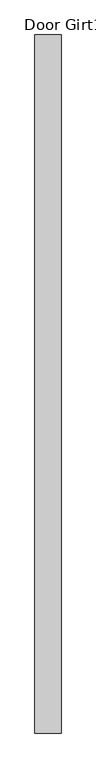
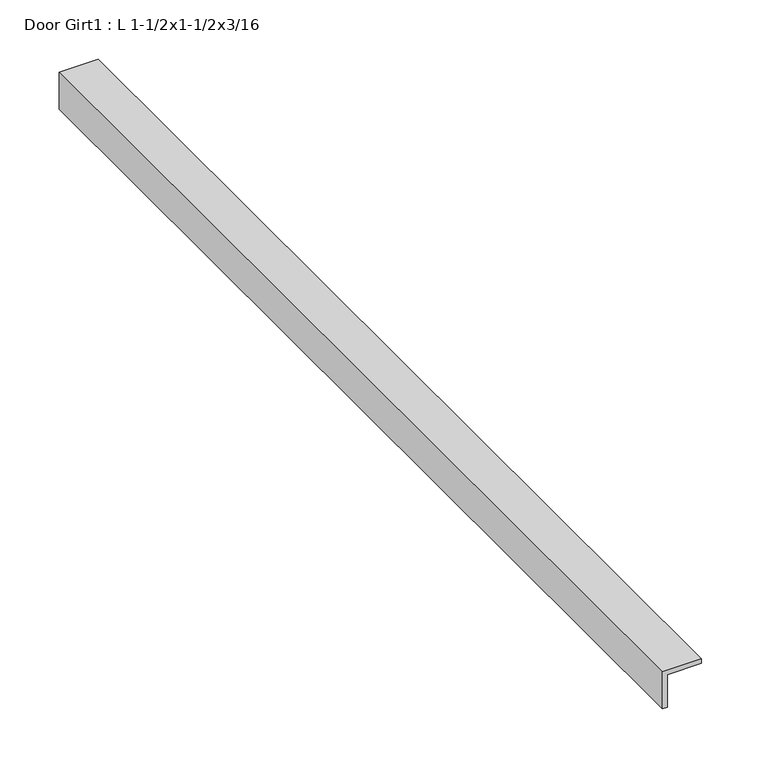
"""IFC4 building model written with IfcOpenShell, lengths in millimetres: proxy geometry, Door Girt1 : L 1-1/2x1-1/2x3/16."""

import ifcopenshell
import ifcopenshell.guid

model = None  # the IFC model being written
_history = None  # IfcOwnerHistory: only IFC2X3 demands one
_inside = {}  # id of a spatial element -> (the spatial element, [elements in it])
_under = {}  # id of a project, library or spatial element -> (it, [spatial elements below it])
_declared = {}  # id of a project -> (the project, [libraries it declares])
_typed = {}  # id of a type object -> (the type object, [elements of that type])
_made_of = {}  # id of a material, layer set ... -> (it, [elements and type objects made of it])


def new_model(schema):
    """Start an empty IFC model of exactly this schema.

    Asked for "IFC4X3", IfcOpenShell would pick the latest addendum, in which some entities
    have other attributes; the version numbers below select the first issue.
    IFC2X3 requires an IfcOwnerHistory on every rooted entity: one is made here for all.
    """
    global model, _history
    if schema == "IFC4X3":
        model = ifcopenshell.file(schema_version=(4, 3, 0, 0))
    else:
        model = ifcopenshell.file(schema=schema)
    _inside.clear()
    _under.clear()
    _declared.clear()
    _typed.clear()
    _made_of.clear()
    _history = None
    if model.schema == "IFC2X3":
        org = make("IfcOrganization", Name="unknown")
        user = make(
            "IfcPersonAndOrganization",
            ThePerson=make("IfcPerson", FamilyName="unknown"),
            TheOrganization=org,
        )
        app = make(
            "IfcApplication",
            ApplicationDeveloper=org,
            Version="unknown",
            ApplicationFullName="unknown",
            ApplicationIdentifier="unknown",
        )
        _history = make(
            "IfcOwnerHistory",
            OwningUser=user,
            OwningApplication=app,
            ChangeAction="ADDED",
            CreationDate=0,
        )
    return model


def make(cls, **values):
    """One entity of the class cls with the attributes given. An attribute that is None is left unset."""
    return model.create_entity(
        cls, **{name: value for name, value in values.items() if value is not None}
    )


def rooted(cls, **values):
    """An entity with a GlobalId (a new one), such as an element, a storey or a relation."""
    return make(cls, GlobalId=ifcopenshell.guid.new(), OwnerHistory=_history, **values)


def si_unit(unit_type, name, prefix=None):
    """IfcSIUnit, for example si_unit("LENGTHUNIT", "METRE", prefix="MILLI")."""
    return make("IfcSIUnit", UnitType=unit_type, Prefix=prefix, Name=name)


def assignment(units):
    """IfcUnitAssignment: the units of a project."""
    return None if units is None else make("IfcUnitAssignment", Units=units)


def point(xyz):
    """IfcCartesianPoint."""
    return None if xyz is None else make("IfcCartesianPoint", Coordinates=xyz)


def direction(xyz):
    """IfcDirection."""
    return None if xyz is None else make("IfcDirection", DirectionRatios=xyz)


def frame(location, z_axis=None, x_axis=None):
    """IfcAxis2Placement3D, a coordinate frame: its origin and axes. An axis left out is left unset."""
    return make(
        "IfcAxis2Placement3D",
        Location=point(location),
        Axis=direction(z_axis),
        RefDirection=direction(x_axis),
    )


def origin():
    """The frame at (0, 0, 0) with its axes left unset."""
    return frame((0.0, 0.0, 0.0))


def place(relative_to, where):
    """IfcLocalPlacement: puts the frame where relative to a parent placement (None: the world)."""
    return make(
        "IfcLocalPlacement", PlacementRelTo=relative_to, RelativePlacement=where
    )


def context(
    kind, dimensions, precision=None, world=None, true_north=None, identifier=None
):
    """IfcGeometricRepresentationContext, for example the 3D "Model" context."""
    return make(
        "IfcGeometricRepresentationContext",
        ContextIdentifier=identifier,
        ContextType=kind,
        CoordinateSpaceDimension=dimensions,
        Precision=precision,
        WorldCoordinateSystem=world,
        TrueNorth=true_north,
    )


def project(units=None, contexts=None):
    """IfcProject with its units and contexts."""
    return rooted(
        "IfcProject",
        Name="project",
        RepresentationContexts=contexts,
        UnitsInContext=assignment(units),
    )


def spatial(cls, under=None, at=None, **own):
    """A site, building, storey or space (cls), placed at a placement, below another one or the project."""
    s = rooted(cls, ObjectPlacement=at, **own)
    if under is not None:
        _under.setdefault(under.id(), (under, []))[1].append(s)
    return s


def polyline(points):
    """IfcPolyline through the points."""
    return make("IfcPolyline", Points=[point(p) for p in points])


def outline(outer, holes=None, kind="AREA"):
    """IfcArbitraryClosedProfileDef: a profile drawn as a closed curve; with holes, ...WithVoids."""
    if holes is None:
        return make("IfcArbitraryClosedProfileDef", ProfileType=kind, OuterCurve=outer)
    return make(
        "IfcArbitraryProfileDefWithVoids",
        ProfileType=kind,
        OuterCurve=outer,
        InnerCurves=holes,
    )


def extrude(swept, where, along, depth):
    """IfcExtrudedAreaSolid: the profile swept, set in the frame where, extruded along a direction by depth."""
    return make(
        "IfcExtrudedAreaSolid",
        SweptArea=swept,
        Position=where,
        ExtrudedDirection=direction(along),
        Depth=depth,
    )


def shape(context_of_items, identifier, shape_type, items):
    """IfcShapeRepresentation: the items that make up one representation, for example the "Body"."""
    return make(
        "IfcShapeRepresentation",
        ContextOfItems=context_of_items,
        RepresentationIdentifier=identifier,
        RepresentationType=shape_type,
        Items=items,
    )


def source(mapping_origin, context_of_items, identifier, shape_type, items):
    """IfcRepresentationMap: a shape defined once, which mapped items show again and again."""
    return make(
        "IfcRepresentationMap",
        MappingOrigin=mapping_origin,
        MappedRepresentation=shape(context_of_items, identifier, shape_type, items),
    )


def transform(
    local_origin,
    x_axis=None,
    y_axis=None,
    z_axis=None,
    scale=None,
    scale2=None,
    scale3=None,
    uniform=True,
):
    """IfcCartesianTransformationOperator3D, or its non-uniform kind. x_axis, y_axis, z_axis: its Axis1, 2, 3."""
    if uniform:
        return make(
            "IfcCartesianTransformationOperator3D",
            Axis1=direction(x_axis),
            Axis2=direction(y_axis),
            LocalOrigin=point(local_origin),
            Scale=scale,
            Axis3=direction(z_axis),
        )
    return make(
        "IfcCartesianTransformationOperator3DnonUniform",
        Axis1=direction(x_axis),
        Axis2=direction(y_axis),
        LocalOrigin=point(local_origin),
        Scale=scale,
        Axis3=direction(z_axis),
        Scale2=scale2,
        Scale3=scale3,
    )


def mapped(mapping_source, mapping_target):
    """IfcMappedItem: shows the shape of a source again, moved by a transform."""
    return make(
        "IfcMappedItem", MappingSource=mapping_source, MappingTarget=mapping_target
    )


def made_of(thing, what):
    """Note that an element or type object is made of a material, layer set ...; save() writes the relation."""
    if what is not None:
        _made_of.setdefault(what.id(), (what, []))[1].append(thing)
    return thing


def element(
    cls,
    number,
    at=None,
    inside=None,
    cuts=None,
    type_object=None,
    material=None,
    context=None,
    identifier="Body",
    shape_type=None,
    held_by="IfcProductDefinitionShape",
    body=None,
    shapes=None,
    **own,
):
    """One element of the class cls, such as IfcWall. Its Tag is "e" and its number.

    at: its placement. inside: the storey or other place that contains it. cuts: it is an
    opening in that element (IfcRelVoidsElement). A single representation is given by context,
    identifier, shape_type and body (its items); several are given by shapes. held_by: the class
    of the entity that holds the representations. save() writes the other relations.
    """
    e = rooted(cls, Tag="e%d" % number, ObjectPlacement=at, **own)
    if body is not None:
        shapes = [shape(context, identifier, shape_type, body)]
    if shapes is not None:
        e.Representation = make(held_by, Representations=shapes)
    if inside is not None:
        _inside.setdefault(inside.id(), (inside, []))[1].append(e)
    if cuts is not None:
        rooted(
            "IfcRelVoidsElement", RelatingBuildingElement=cuts, RelatedOpeningElement=e
        )
    if type_object is not None:
        _typed.setdefault(type_object.id(), (type_object, []))[1].append(e)
    return made_of(e, material)


def aggregate(whole, parts):
    """IfcRelAggregates: a whole, such as a stair, and the parts it consists of."""
    return rooted("IfcRelAggregates", RelatingObject=whole, RelatedObjects=parts)


def save(model, path):
    """Write the relations noted so far, then the file.

    IfcRelAggregates (storeys below a building ...), IfcRelContainedInSpatialStructure (elements
    in a storey), IfcRelDefinesByType, IfcRelAssociatesMaterial and IfcRelDeclares: one each for
    every whole, place, type object, material and project.
    """
    for whole, parts in _under.values():
        aggregate(whole, parts)
    for where, things in _inside.values():
        rooted(
            "IfcRelContainedInSpatialStructure",
            RelatedElements=things,
            RelatingStructure=where,
        )
    for kind, things in _typed.values():
        rooted("IfcRelDefinesByType", RelatedObjects=things, RelatingType=kind)
    for what, things in _made_of.values():
        rooted("IfcRelAssociatesMaterial", RelatedObjects=things, RelatingMaterial=what)
    for by, libraries in _declared.values():
        rooted("IfcRelDeclares", RelatingContext=by, RelatedDefinitions=libraries)
    model.write(path)


def door_girt1_l_1_1_2x1_1_2x3_16_7802d8c0(model_context):
    return source(origin(), model_context, "Body", "SweptSolid", [
        extrude(outline(polyline([(1625.6, 587403.9934739), (1625.6, 587365.8934739), (1587.5, 587365.8934739), (1587.5, 587370.6559739), (1620.8375, 587370.6559739), (1620.8375, 587403.9934739), (1625.6, 587403.9934739)])), frame((0.0, -535163.4663841, 0.0), z_axis=(0.0, 1.0, 0.0), x_axis=(0.0, 0.0, 1.0)), (0.0, 0.0, 1.0), 1017.5875),
    ])


if __name__ == "__main__":
    model = new_model("IFC4")
    model_context = context("Model", 3, world=origin())
    ifc_project = project(units=[si_unit("LENGTHUNIT", "METRE", prefix="MILLI")], contexts=[model_context])
    site = spatial("IfcSite", under=ifc_project)
    building = spatial("IfcBuilding", under=site)
    placement = place(None, origin())
    door_girt1_l_1_1_2x1_1_2x3_16_shape = door_girt1_l_1_1_2x1_1_2x3_16_7802d8c0(model_context)
    element("IfcBuildingElementProxy", 1, Name="Door Girt1 : L 1-1/2x1-1/2x3/16", ObjectType="Door Girt1 : L 1-1/2x1-1/2x3/16", at=placement, inside=building, context=model_context, shape_type="MappedRepresentation", body=[
        mapped(door_girt1_l_1_1_2x1_1_2x3_16_shape, transform((0.0, 0.0, 0.0), x_axis=(1.0, 0.0, 0.0), y_axis=(0.0, 1.0, 0.0), z_axis=(0.0, 0.0, 1.0))),
    ])
    save(model, "model.ifc")

# Revit data of these elements
# Element 1 (IfcBuildingElementProxy, "Door Girt1 : L 1-1/2x1-1/2x3/16")
#   Materials on its faces: "1-1/2\"X1-1/2\" GALV. STL L"
# Materials
#   "1-1/2\"X1-1/2\" GALV. STL L": class "Generic", colour RGB 211 211 207, transparency 0, Cost = 0
